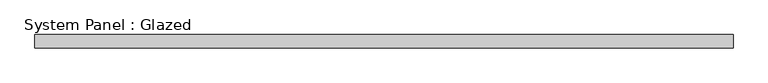
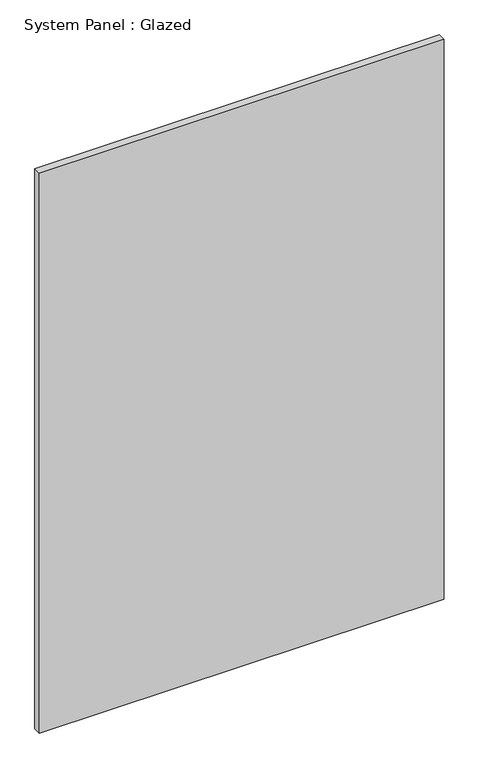
"""IFC4 building model written with IfcOpenShell, lengths in millimetres: plate geometry, System Panel : Glazed."""

import ifcopenshell
import ifcopenshell.guid

model = None  # the IFC model being written
_history = None  # IfcOwnerHistory: only IFC2X3 demands one
_inside = {}  # id of a spatial element -> (the spatial element, [elements in it])
_under = {}  # id of a project, library or spatial element -> (it, [spatial elements below it])
_declared = {}  # id of a project -> (the project, [libraries it declares])
_typed = {}  # id of a type object -> (the type object, [elements of that type])
_made_of = {}  # id of a material, layer set ... -> (it, [elements and type objects made of it])


def new_model(schema):
    """Start an empty IFC model of exactly this schema.

    Asked for "IFC4X3", IfcOpenShell would pick the latest addendum, in which some entities
    have other attributes; the version numbers below select the first issue.
    IFC2X3 requires an IfcOwnerHistory on every rooted entity: one is made here for all.
    """
    global model, _history
    if schema == "IFC4X3":
        model = ifcopenshell.file(schema_version=(4, 3, 0, 0))
    else:
        model = ifcopenshell.file(schema=schema)
    _inside.clear()
    _under.clear()
    _declared.clear()
    _typed.clear()
    _made_of.clear()
    _history = None
    if model.schema == "IFC2X3":
        org = make("IfcOrganization", Name="unknown")
        user = make(
            "IfcPersonAndOrganization",
            ThePerson=make("IfcPerson", FamilyName="unknown"),
            TheOrganization=org,
        )
        app = make(
            "IfcApplication",
            ApplicationDeveloper=org,
            Version="unknown",
            ApplicationFullName="unknown",
            ApplicationIdentifier="unknown",
        )
        _history = make(
            "IfcOwnerHistory",
            OwningUser=user,
            OwningApplication=app,
            ChangeAction="ADDED",
            CreationDate=0,
        )
    return model


def make(cls, **values):
    """One entity of the class cls with the attributes given. An attribute that is None is left unset."""
    return model.create_entity(
        cls, **{name: value for name, value in values.items() if value is not None}
    )


def rooted(cls, **values):
    """An entity with a GlobalId (a new one), such as an element, a storey or a relation."""
    return make(cls, GlobalId=ifcopenshell.guid.new(), OwnerHistory=_history, **values)


def si_unit(unit_type, name, prefix=None):
    """IfcSIUnit, for example si_unit("LENGTHUNIT", "METRE", prefix="MILLI")."""
    return make("IfcSIUnit", UnitType=unit_type, Prefix=prefix, Name=name)


def assignment(units):
    """IfcUnitAssignment: the units of a project."""
    return None if units is None else make("IfcUnitAssignment", Units=units)


def point(xyz):
    """IfcCartesianPoint."""
    return None if xyz is None else make("IfcCartesianPoint", Coordinates=xyz)


def direction(xyz):
    """IfcDirection."""
    return None if xyz is None else make("IfcDirection", DirectionRatios=xyz)


def frame(location, z_axis=None, x_axis=None):
    """IfcAxis2Placement3D, a coordinate frame: its origin and axes. An axis left out is left unset."""
    return make(
        "IfcAxis2Placement3D",
        Location=point(location),
        Axis=direction(z_axis),
        RefDirection=direction(x_axis),
    )


def origin():
    """The frame at (0, 0, 0) with its axes left unset."""
    return frame((0.0, 0.0, 0.0))


def origin_with_axes():
    """The frame at (0, 0, 0) with the z axis (0, 0, 1) and the x axis (1, 0, 0) written out."""
    return frame((0.0, 0.0, 0.0), z_axis=(0.0, 0.0, 1.0), x_axis=(1.0, 0.0, 0.0))


def place(relative_to, where):
    """IfcLocalPlacement: puts the frame where relative to a parent placement (None: the world)."""
    return make(
        "IfcLocalPlacement", PlacementRelTo=relative_to, RelativePlacement=where
    )


def context(
    kind, dimensions, precision=None, world=None, true_north=None, identifier=None
):
    """IfcGeometricRepresentationContext, for example the 3D "Model" context."""
    return make(
        "IfcGeometricRepresentationContext",
        ContextIdentifier=identifier,
        ContextType=kind,
        CoordinateSpaceDimension=dimensions,
        Precision=precision,
        WorldCoordinateSystem=world,
        TrueNorth=true_north,
    )


def project(units=None, contexts=None):
    """IfcProject with its units and contexts."""
    return rooted(
        "IfcProject",
        Name="project",
        RepresentationContexts=contexts,
        UnitsInContext=assignment(units),
    )


def spatial(cls, under=None, at=None, **own):
    """A site, building, storey or space (cls), placed at a placement, below another one or the project."""
    s = rooted(cls, ObjectPlacement=at, **own)
    if under is not None:
        _under.setdefault(under.id(), (under, []))[1].append(s)
    return s


def polyline(points):
    """IfcPolyline through the points."""
    return make("IfcPolyline", Points=[point(p) for p in points])


def outline(outer, holes=None, kind="AREA"):
    """IfcArbitraryClosedProfileDef: a profile drawn as a closed curve; with holes, ...WithVoids."""
    if holes is None:
        return make("IfcArbitraryClosedProfileDef", ProfileType=kind, OuterCurve=outer)
    return make(
        "IfcArbitraryProfileDefWithVoids",
        ProfileType=kind,
        OuterCurve=outer,
        InnerCurves=holes,
    )


def extrude(swept, where, along, depth):
    """IfcExtrudedAreaSolid: the profile swept, set in the frame where, extruded along a direction by depth."""
    return make(
        "IfcExtrudedAreaSolid",
        SweptArea=swept,
        Position=where,
        ExtrudedDirection=direction(along),
        Depth=depth,
    )


def shape(context_of_items, identifier, shape_type, items):
    """IfcShapeRepresentation: the items that make up one representation, for example the "Body"."""
    return make(
        "IfcShapeRepresentation",
        ContextOfItems=context_of_items,
        RepresentationIdentifier=identifier,
        RepresentationType=shape_type,
        Items=items,
    )


def source(mapping_origin, context_of_items, identifier, shape_type, items):
    """IfcRepresentationMap: a shape defined once, which mapped items show again and again."""
    return make(
        "IfcRepresentationMap",
        MappingOrigin=mapping_origin,
        MappedRepresentation=shape(context_of_items, identifier, shape_type, items),
    )


def transform(
    local_origin,
    x_axis=None,
    y_axis=None,
    z_axis=None,
    scale=None,
    scale2=None,
    scale3=None,
    uniform=True,
):
    """IfcCartesianTransformationOperator3D, or its non-uniform kind. x_axis, y_axis, z_axis: its Axis1, 2, 3."""
    if uniform:
        return make(
            "IfcCartesianTransformationOperator3D",
            Axis1=direction(x_axis),
            Axis2=direction(y_axis),
            LocalOrigin=point(local_origin),
            Scale=scale,
            Axis3=direction(z_axis),
        )
    return make(
        "IfcCartesianTransformationOperator3DnonUniform",
        Axis1=direction(x_axis),
        Axis2=direction(y_axis),
        LocalOrigin=point(local_origin),
        Scale=scale,
        Axis3=direction(z_axis),
        Scale2=scale2,
        Scale3=scale3,
    )


def mapped(mapping_source, mapping_target):
    """IfcMappedItem: shows the shape of a source again, moved by a transform."""
    return make(
        "IfcMappedItem", MappingSource=mapping_source, MappingTarget=mapping_target
    )


def made_of(thing, what):
    """Note that an element or type object is made of a material, layer set ...; save() writes the relation."""
    if what is not None:
        _made_of.setdefault(what.id(), (what, []))[1].append(thing)
    return thing


def element(
    cls,
    number,
    at=None,
    inside=None,
    cuts=None,
    type_object=None,
    material=None,
    context=None,
    identifier="Body",
    shape_type=None,
    held_by="IfcProductDefinitionShape",
    body=None,
    shapes=None,
    **own,
):
    """One element of the class cls, such as IfcWall. Its Tag is "e" and its number.

    at: its placement. inside: the storey or other place that contains it. cuts: it is an
    opening in that element (IfcRelVoidsElement). A single representation is given by context,
    identifier, shape_type and body (its items); several are given by shapes. held_by: the class
    of the entity that holds the representations. save() writes the other relations.
    """
    e = rooted(cls, Tag="e%d" % number, ObjectPlacement=at, **own)
    if body is not None:
        shapes = [shape(context, identifier, shape_type, body)]
    if shapes is not None:
        e.Representation = make(held_by, Representations=shapes)
    if inside is not None:
        _inside.setdefault(inside.id(), (inside, []))[1].append(e)
    if cuts is not None:
        rooted(
            "IfcRelVoidsElement", RelatingBuildingElement=cuts, RelatedOpeningElement=e
        )
    if type_object is not None:
        _typed.setdefault(type_object.id(), (type_object, []))[1].append(e)
    return made_of(e, material)


def aggregate(whole, parts):
    """IfcRelAggregates: a whole, such as a stair, and the parts it consists of."""
    return rooted("IfcRelAggregates", RelatingObject=whole, RelatedObjects=parts)


def save(model, path):
    """Write the relations noted so far, then the file.

    IfcRelAggregates (storeys below a building ...), IfcRelContainedInSpatialStructure (elements
    in a storey), IfcRelDefinesByType, IfcRelAssociatesMaterial and IfcRelDeclares: one each for
    every whole, place, type object, material and project.
    """
    for whole, parts in _under.values():
        aggregate(whole, parts)
    for where, things in _inside.values():
        rooted(
            "IfcRelContainedInSpatialStructure",
            RelatedElements=things,
            RelatingStructure=where,
        )
    for kind, things in _typed.values():
        rooted("IfcRelDefinesByType", RelatedObjects=things, RelatingType=kind)
    for what, things in _made_of.values():
        rooted("IfcRelAssociatesMaterial", RelatedObjects=things, RelatingMaterial=what)
    for by, libraries in _declared.values():
        rooted("IfcRelDeclares", RelatingContext=by, RelatedDefinitions=libraries)
    model.write(path)


def system_panel_glazed_41482947(model_context):
    return source(origin(), model_context, "Body", "SweptSolid", [
        extrude(outline(polyline([(669.7103534, 19.05), (-669.7103534, 19.05), (-669.7103534, 44.45), (669.7103534, 44.45), (669.7103534, 19.05)])), origin_with_axes(), (0.0, 0.0, 1.0), 1957.9166667),
    ])


if __name__ == "__main__":
    model = new_model("IFC4")
    model_context = context("Model", 3, world=origin())
    ifc_project = project(units=[si_unit("LENGTHUNIT", "METRE", prefix="MILLI")], contexts=[model_context])
    site = spatial("IfcSite", under=ifc_project)
    building = spatial("IfcBuilding", under=site)
    placement = place(None, origin())
    system_panel_glazed_shape = system_panel_glazed_41482947(model_context)
    element("IfcPlate", 1, ObjectType="System Panel : Glazed", at=placement, inside=building, context=model_context, shape_type="MappedRepresentation", body=[
        mapped(system_panel_glazed_shape, transform((0.0, 0.0, 0.0), x_axis=(1.0, 0.0, 0.0), y_axis=(0.0, 1.0, 0.0), z_axis=(0.0, 0.0, 1.0))),
    ])
    save(model, "model.ifc")

# Revit data of these elements
# Type "System Panel : Glazed"
#   Construction Type Id = "GSP4R"
#   Analytic Construction = "1/8 in Pilkington single glazing"
#   Visual Light Transmittance = 0.9
#   Solar Heat Gain Coefficient = 0.86
#   Heat Transfer Coefficient (U) = 1.18115 BTU/(h·ft²·°F)
#   Define Thermal Properties by = 1
# Element 1 (IfcPlate, "System Panel : Glazed")
#   Materials on its faces: "Glass"
# Materials
#   "Glass": class "Glass", colour RGB 0 128 192, transparency 0.75, Description = "Soda Lime Glass", Cost = 0
